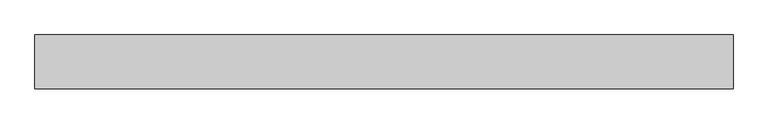
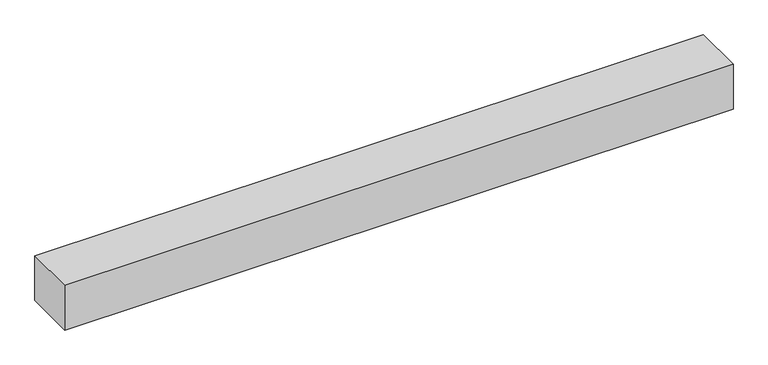
"""IFC4 building model written with IfcOpenShell, lengths in millimetres: proxy geometry, Framing058 2488 : Framing058 2488."""

from ifc_helpers import new_model, si_unit, frame, origin, place, context, project, spatial, polyline, outline, extrude, source, transform, mapped, element, save


def generic_models_7c2a7588(model_context):
    return source(origin(), model_context, "Body", "SweptSolid", [
        extrude(outline(polyline([(-718.8864422, 794.7093426), (-2694.3737014, 794.7093426), (-2694.3737014, 947.1093426), (-718.8864422, 947.1093426), (-718.8864422, 794.7093426)])), frame((0.0, 0.0, 39579.2960083), z_axis=(0.0, 0.0, 1.0), x_axis=(1.0, 0.0, 0.0)), (0.0, 0.0, 1.0), 139.7),
    ])


if __name__ == "__main__":
    model = new_model("IFC4")
    model_context = context("Model", 3, world=origin())
    ifc_project = project(units=[si_unit("LENGTHUNIT", "METRE", prefix="MILLI")], contexts=[model_context])
    site = spatial("IfcSite", under=ifc_project)
    building = spatial("IfcBuilding", under=site)
    placement = place(None, origin())
    generic_models_shape = generic_models_7c2a7588(model_context)
    element("IfcBuildingElementProxy", 1, Name="Framing058 2488 : Framing058 2488", ObjectType="Framing058 2488 : Framing058 2488", at=placement, inside=building, context=model_context, shape_type="MappedRepresentation", body=[
        mapped(generic_models_shape, transform((0.0, 0.0, 0.0), x_axis=(1.0, 0.0, 0.0), y_axis=(0.0, 1.0, 0.0), z_axis=(0.0, 0.0, 1.0))),
    ])
    save(model, "model.ifc")

# Revit data of these elements
# Type "Framing058 2488 : Framing058 2488"
#   NameOverride = "Framing058"
# Element 1 (IfcBuildingElementProxy, "Framing058 2488 : Framing058 2488")
#   Materials on its faces: "WOOD FRAMING (SEE STRUCT DWGS)"
# Materials
#   "WOOD FRAMING (SEE STRUCT DWGS)": class "Unassigned", colour RGB 224 188 168, transparency 0, Cost = 0
